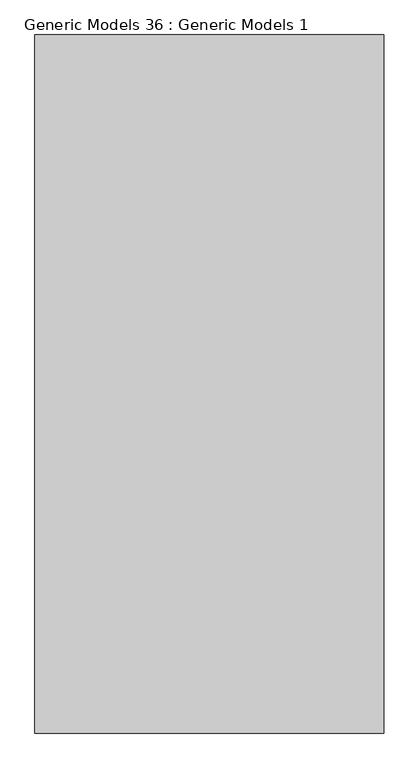
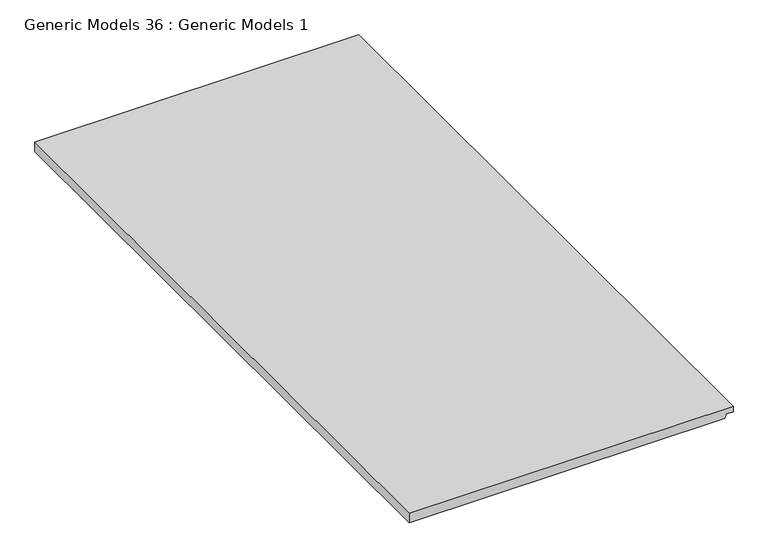
"""IFC4 building model written with IfcOpenShell, lengths in millimetres: proxy geometry, Generic Models 36 : Generic Models 1."""

import ifcopenshell
import ifcopenshell.guid

model = None  # the IFC model being written
_history = None  # IfcOwnerHistory: only IFC2X3 demands one
_inside = {}  # id of a spatial element -> (the spatial element, [elements in it])
_under = {}  # id of a project, library or spatial element -> (it, [spatial elements below it])
_declared = {}  # id of a project -> (the project, [libraries it declares])
_typed = {}  # id of a type object -> (the type object, [elements of that type])
_made_of = {}  # id of a material, layer set ... -> (it, [elements and type objects made of it])


def new_model(schema):
    """Start an empty IFC model of exactly this schema.

    Asked for "IFC4X3", IfcOpenShell would pick the latest addendum, in which some entities
    have other attributes; the version numbers below select the first issue.
    IFC2X3 requires an IfcOwnerHistory on every rooted entity: one is made here for all.
    """
    global model, _history
    if schema == "IFC4X3":
        model = ifcopenshell.file(schema_version=(4, 3, 0, 0))
    else:
        model = ifcopenshell.file(schema=schema)
    _inside.clear()
    _under.clear()
    _declared.clear()
    _typed.clear()
    _made_of.clear()
    _history = None
    if model.schema == "IFC2X3":
        org = make("IfcOrganization", Name="unknown")
        user = make(
            "IfcPersonAndOrganization",
            ThePerson=make("IfcPerson", FamilyName="unknown"),
            TheOrganization=org,
        )
        app = make(
            "IfcApplication",
            ApplicationDeveloper=org,
            Version="unknown",
            ApplicationFullName="unknown",
            ApplicationIdentifier="unknown",
        )
        _history = make(
            "IfcOwnerHistory",
            OwningUser=user,
            OwningApplication=app,
            ChangeAction="ADDED",
            CreationDate=0,
        )
    return model


def make(cls, **values):
    """One entity of the class cls with the attributes given. An attribute that is None is left unset."""
    return model.create_entity(
        cls, **{name: value for name, value in values.items() if value is not None}
    )


def rooted(cls, **values):
    """An entity with a GlobalId (a new one), such as an element, a storey or a relation."""
    return make(cls, GlobalId=ifcopenshell.guid.new(), OwnerHistory=_history, **values)


def si_unit(unit_type, name, prefix=None):
    """IfcSIUnit, for example si_unit("LENGTHUNIT", "METRE", prefix="MILLI")."""
    return make("IfcSIUnit", UnitType=unit_type, Prefix=prefix, Name=name)


def assignment(units):
    """IfcUnitAssignment: the units of a project."""
    return None if units is None else make("IfcUnitAssignment", Units=units)


def point(xyz):
    """IfcCartesianPoint."""
    return None if xyz is None else make("IfcCartesianPoint", Coordinates=xyz)


def direction(xyz):
    """IfcDirection."""
    return None if xyz is None else make("IfcDirection", DirectionRatios=xyz)


def frame(location, z_axis=None, x_axis=None):
    """IfcAxis2Placement3D, a coordinate frame: its origin and axes. An axis left out is left unset."""
    return make(
        "IfcAxis2Placement3D",
        Location=point(location),
        Axis=direction(z_axis),
        RefDirection=direction(x_axis),
    )


def origin():
    """The frame at (0, 0, 0) with its axes left unset."""
    return frame((0.0, 0.0, 0.0))


def place(relative_to, where):
    """IfcLocalPlacement: puts the frame where relative to a parent placement (None: the world)."""
    return make(
        "IfcLocalPlacement", PlacementRelTo=relative_to, RelativePlacement=where
    )


def context(
    kind, dimensions, precision=None, world=None, true_north=None, identifier=None
):
    """IfcGeometricRepresentationContext, for example the 3D "Model" context."""
    return make(
        "IfcGeometricRepresentationContext",
        ContextIdentifier=identifier,
        ContextType=kind,
        CoordinateSpaceDimension=dimensions,
        Precision=precision,
        WorldCoordinateSystem=world,
        TrueNorth=true_north,
    )


def project(units=None, contexts=None):
    """IfcProject with its units and contexts."""
    return rooted(
        "IfcProject",
        Name="project",
        RepresentationContexts=contexts,
        UnitsInContext=assignment(units),
    )


def spatial(cls, under=None, at=None, **own):
    """A site, building, storey or space (cls), placed at a placement, below another one or the project."""
    s = rooted(cls, ObjectPlacement=at, **own)
    if under is not None:
        _under.setdefault(under.id(), (under, []))[1].append(s)
    return s


def polyline(points):
    """IfcPolyline through the points."""
    return make("IfcPolyline", Points=[point(p) for p in points])


def outline(outer, holes=None, kind="AREA"):
    """IfcArbitraryClosedProfileDef: a profile drawn as a closed curve; with holes, ...WithVoids."""
    if holes is None:
        return make("IfcArbitraryClosedProfileDef", ProfileType=kind, OuterCurve=outer)
    return make(
        "IfcArbitraryProfileDefWithVoids",
        ProfileType=kind,
        OuterCurve=outer,
        InnerCurves=holes,
    )


def extrude(swept, where, along, depth):
    """IfcExtrudedAreaSolid: the profile swept, set in the frame where, extruded along a direction by depth."""
    return make(
        "IfcExtrudedAreaSolid",
        SweptArea=swept,
        Position=where,
        ExtrudedDirection=direction(along),
        Depth=depth,
    )


def shape(context_of_items, identifier, shape_type, items):
    """IfcShapeRepresentation: the items that make up one representation, for example the "Body"."""
    return make(
        "IfcShapeRepresentation",
        ContextOfItems=context_of_items,
        RepresentationIdentifier=identifier,
        RepresentationType=shape_type,
        Items=items,
    )


def source(mapping_origin, context_of_items, identifier, shape_type, items):
    """IfcRepresentationMap: a shape defined once, which mapped items show again and again."""
    return make(
        "IfcRepresentationMap",
        MappingOrigin=mapping_origin,
        MappedRepresentation=shape(context_of_items, identifier, shape_type, items),
    )


def transform(
    local_origin,
    x_axis=None,
    y_axis=None,
    z_axis=None,
    scale=None,
    scale2=None,
    scale3=None,
    uniform=True,
):
    """IfcCartesianTransformationOperator3D, or its non-uniform kind. x_axis, y_axis, z_axis: its Axis1, 2, 3."""
    if uniform:
        return make(
            "IfcCartesianTransformationOperator3D",
            Axis1=direction(x_axis),
            Axis2=direction(y_axis),
            LocalOrigin=point(local_origin),
            Scale=scale,
            Axis3=direction(z_axis),
        )
    return make(
        "IfcCartesianTransformationOperator3DnonUniform",
        Axis1=direction(x_axis),
        Axis2=direction(y_axis),
        LocalOrigin=point(local_origin),
        Scale=scale,
        Axis3=direction(z_axis),
        Scale2=scale2,
        Scale3=scale3,
    )


def mapped(mapping_source, mapping_target):
    """IfcMappedItem: shows the shape of a source again, moved by a transform."""
    return make(
        "IfcMappedItem", MappingSource=mapping_source, MappingTarget=mapping_target
    )


def made_of(thing, what):
    """Note that an element or type object is made of a material, layer set ...; save() writes the relation."""
    if what is not None:
        _made_of.setdefault(what.id(), (what, []))[1].append(thing)
    return thing


def element(
    cls,
    number,
    at=None,
    inside=None,
    cuts=None,
    type_object=None,
    material=None,
    context=None,
    identifier="Body",
    shape_type=None,
    held_by="IfcProductDefinitionShape",
    body=None,
    shapes=None,
    **own,
):
    """One element of the class cls, such as IfcWall. Its Tag is "e" and its number.

    at: its placement. inside: the storey or other place that contains it. cuts: it is an
    opening in that element (IfcRelVoidsElement). A single representation is given by context,
    identifier, shape_type and body (its items); several are given by shapes. held_by: the class
    of the entity that holds the representations. save() writes the other relations.
    """
    e = rooted(cls, Tag="e%d" % number, ObjectPlacement=at, **own)
    if body is not None:
        shapes = [shape(context, identifier, shape_type, body)]
    if shapes is not None:
        e.Representation = make(held_by, Representations=shapes)
    if inside is not None:
        _inside.setdefault(inside.id(), (inside, []))[1].append(e)
    if cuts is not None:
        rooted(
            "IfcRelVoidsElement", RelatingBuildingElement=cuts, RelatedOpeningElement=e
        )
    if type_object is not None:
        _typed.setdefault(type_object.id(), (type_object, []))[1].append(e)
    return made_of(e, material)


def aggregate(whole, parts):
    """IfcRelAggregates: a whole, such as a stair, and the parts it consists of."""
    return rooted("IfcRelAggregates", RelatingObject=whole, RelatedObjects=parts)


def save(model, path):
    """Write the relations noted so far, then the file.

    IfcRelAggregates (storeys below a building ...), IfcRelContainedInSpatialStructure (elements
    in a storey), IfcRelDefinesByType, IfcRelAssociatesMaterial and IfcRelDeclares: one each for
    every whole, place, type object, material and project.
    """
    for whole, parts in _under.values():
        aggregate(whole, parts)
    for where, things in _inside.values():
        rooted(
            "IfcRelContainedInSpatialStructure",
            RelatedElements=things,
            RelatingStructure=where,
        )
    for kind, things in _typed.values():
        rooted("IfcRelDefinesByType", RelatedObjects=things, RelatingType=kind)
    for what, things in _made_of.values():
        rooted("IfcRelAssociatesMaterial", RelatedObjects=things, RelatingMaterial=what)
    for by, libraries in _declared.values():
        rooted("IfcRelDeclares", RelatingContext=by, RelatedDefinitions=libraries)
    model.write(path)


def generic_models_36_generic_models_1_28f40251(model_context):
    return source(origin(), model_context, "Body", "SweptSolid", [
        extrude(outline(polyline([(2253.330428, 49662.5798593), (2253.330428, 49052.9798593), (2234.280428, 49052.9798593), (2234.280428, 49646.9908455), (2242.217928, 49649.8798593), (2242.217928, 49662.5798593), (2253.330428, 49662.5798593)])), frame((0.0, 0.0, 0.0), z_axis=(0.0, 1.0, 0.0), x_axis=(0.0, 0.0, 1.0)), (0.0, 0.0, 1.0), 1219.2),
    ])


if __name__ == "__main__":
    model = new_model("IFC4")
    model_context = context("Model", 3, world=origin())
    ifc_project = project(units=[si_unit("LENGTHUNIT", "METRE", prefix="MILLI")], contexts=[model_context])
    site = spatial("IfcSite", under=ifc_project)
    building = spatial("IfcBuilding", under=site)
    placement = place(None, origin())
    generic_models_36_generic_models_1_shape = generic_models_36_generic_models_1_28f40251(model_context)
    element("IfcBuildingElementProxy", 1, Name="Generic Models 36 : Generic Models 1", ObjectType="Generic Models 36 : Generic Models 1", at=placement, inside=building, context=model_context, shape_type="MappedRepresentation", body=[
        mapped(generic_models_36_generic_models_1_shape, transform((0.0, 0.0, 0.0), x_axis=(1.0, 0.0, 0.0), y_axis=(0.0, 1.0, 0.0), z_axis=(0.0, 0.0, 1.0))),
    ])
    save(model, "model.ifc")

# Revit data of these elements
# Project information
#   Project Issue Date = "Issue Date"
#   Project Status = "Project Status"
#   Client Name = "Owner"
#   Project Address = "Enter address here"
#   Project Name = "Project Name"
#   Project Number = "Project Number"
# Element 1 (IfcBuildingElementProxy, "Generic Models 36 : Generic Models 1")
#   Materials on its faces: "CEILING AS SCHEDULED"
# Materials
#   "CEILING AS SCHEDULED": class "Generic", colour RGB 255 255 255, transparency 0, Cost = 0
